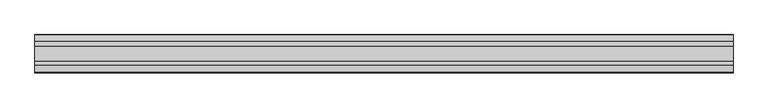
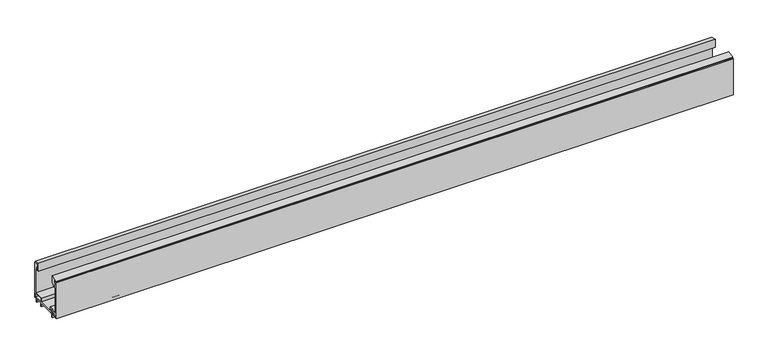
"""IFC4 building model written with IfcOpenShell, lengths in millimetres: proxy geometry, Generic Models 3:Generic Models 2:312240:Generic Models 2:312240 : Generic Models 3:Generic Models 2:312240:21 : Generic Models 3:Generic Models 2:312240:Generic Models 2:312240 : Generic Models 3:Generic Models 2:312240:300533."""

from ifc_helpers import new_model, si_unit, frame, origin, place, context, project, spatial, polyline, outline, extrude, source, transform, mapped, element, save


def generic_models_bb2c0e95(model_context):
    return source(origin(), model_context, "Body", "SweptSolid", [
        extrude(outline(polyline([(-579089.3927119, 38.4543134), (-579089.3434673, 37.5044445), (-579090.0840224, 37.0107412), (-579091.0973491, 37.6694036), (-579092.5052258, 37.6694036), (-579092.5052258, 35.3570787), (-579095.6476161, 35.3570787), (-579095.6476161, 99.8650152), (-579090.1929009, 99.8650152), (-579090.1929009, 96.7226249), (-579091.9716123, 96.426173), (-579090.1929009, 91.5643616), (-579090.1929009, 87.295454), (-579092.5052258, 87.295454), (-579092.5052258, 42.7683765), (-579080.3506973, 42.7683765), (-579080.3506973, 41.3962277), (-579090.2521912, 39.9817285), (-579090.2521912, 38.9309415), (-579089.3927119, 38.4543134)])), frame((591598.4983953, 0.0, 0.0), z_axis=(1.0, 0.0, 0.0), x_axis=(0.0, 1.0, 0.0)), (0.0, 0.0, 1.0), 1150.6736578),
        extrude(outline(polyline([(-579094.0351774, 101.101348), (-579082.6037319, 104.1497335), (-579082.6037319, 92.5441205), (-579088.6970113, 87.295454), (-579089.9023153, 87.295454), (-579089.9023153, 91.8245902), (-579091.4443521, 96.039491), (-579089.9023153, 96.2964971), (-579089.9023153, 100.0627349), (-579094.0351774, 100.0627349), (-579094.0351774, 101.101348)])), frame((591598.4983953, 0.0, 0.0), z_axis=(1.0, 0.0, 0.0), x_axis=(0.0, 1.0, 0.0)), (0.0, 0.0, 1.0), 1150.6736578),
        extrude(outline(polyline([(-579034.6971025, 88.0069386), (-579039.262462, 88.0069386), (-579039.262462, 90.0525332), (-579037.9580736, 91.3568057), (-579037.9580736, 89.5484886), (-579036.475814, 89.5484886), (-579035.4819937, 91.2698359), (-579035.4819937, 93.551255), (-579036.3674154, 95.450048), (-579037.9580736, 95.450048), (-579037.9580736, 93.4168245), (-579039.262462, 93.639525), (-579039.262462, 98.6792075), (-579032.1476161, 98.0807625), (-579032.1476161, 35.6535306), (-579035.7050391, 35.6535306), (-579035.7050391, 29.36875), (-579037.7209121, 29.36875), (-579037.7209121, 35.6535306), (-579048.6303425, 35.6535306), (-579048.6303425, 29.36875), (-579050.6462155, 29.36875), (-579050.6462155, 35.6535306), (-579081.7143761, 35.6535306), (-579081.7143761, 29.36875), (-579083.7302491, 29.36875), (-579083.7302491, 35.6535306), (-579092.3273546, 35.6535306), (-579092.3273546, 37.0172094), (-579091.4972893, 37.5508228), (-579090.5486432, 36.8986286), (-579083.7302491, 36.8986286), (-579082.4258607, 38.203017), (-579078.6905666, 38.203017), (-579078.6905666, 43.5391515), (-579092.1494835, 43.5391515), (-579092.1494835, 45.0807014), (-579076.6746936, 45.0807014), (-579076.6746936, 38.203017), (-579050.7647963, 38.203017), (-579050.7647963, 45.0807014), (-579034.6971025, 45.0807014), (-579034.6971025, 88.0069386)]), holes=[polyline([(-579035.2900064, 37.7879844), (-579035.2900064, 43.5391515), (-579048.6303425, 43.5391515), (-579048.6303425, 37.7879844), (-579035.2900064, 37.7879844)])]), frame((591598.4983953, 0.0, 0.0), z_axis=(1.0, 0.0, 0.0), x_axis=(0.0, 1.0, 0.0)), (0.0, 0.0, 1.0), 1150.6736578),
        extrude(outline(polyline([(-579042.6037319, 102.6595575), (-579032.6450924, 100.4407933), (-579032.6450924, 98.3393783), (-579039.5693075, 98.9217889), (-579039.5693075, 93.4814891), (-579037.6456554, 93.1530607), (-579037.6456554, 95.1913241), (-579036.6213064, 95.1913241), (-579035.7812608, 93.3898405), (-579035.7812608, 91.309542), (-579036.6417092, 89.8192017), (-579037.7308961, 89.8192017), (-579037.7308961, 92.0735899), (-579039.5693075, 90.2351786), (-579039.5693075, 88.0069386), (-579042.6037319, 88.0069386), (-579042.6037319, 102.6595575)])), frame((591598.4983953, 0.0, 0.0), z_axis=(1.0, 0.0, 0.0), x_axis=(0.0, 1.0, 0.0)), (0.0, 0.0, 1.0), 1150.6736578),
    ])


if __name__ == "__main__":
    model = new_model("IFC4")
    model_context = context("Model", 3, world=origin())
    ifc_project = project(units=[si_unit("LENGTHUNIT", "METRE", prefix="MILLI")], contexts=[model_context])
    site = spatial("IfcSite", under=ifc_project)
    building = spatial("IfcBuilding", under=site)
    placement = place(None, origin())
    generic_models_shape = generic_models_bb2c0e95(model_context)
    element("IfcBuildingElementProxy", 1, Name="Generic Models 3:Generic Models 2:312240:Generic Models 2:312240 : Generic Models 3:Generic Models 2:312240:21 : Generic Models 3:Generic Models 2:312240:Generic Models 2:312240 : Generic Models 3:Generic Models 2:312240:300533", ObjectType="Generic Models 3:Generic Models 2:312240:Generic Models 2:312240 : Generic Models 3:Generic Models 2:312240:21 : Generic Models 3:Generic Models 2:312240:Generic Models 2:312240 : Generic Models 3:Generic Models 2:312240:300533", at=placement, inside=building, context=model_context, shape_type="MappedRepresentation", body=[
        mapped(generic_models_shape, transform((0.0, 0.0, 0.0), x_axis=(1.0, 0.0, 0.0), y_axis=(0.0, 1.0, 0.0), z_axis=(0.0, 0.0, 1.0))),
    ])
    save(model, "model.ifc")

# Revit data of these elements
# Type "Generic Models 3:Generic Models 2:312240:Generic Models 2:312240 : Generic Models 3:Generic Models 2:312240:21 : Generic Models 3:Generic Models 2:312240:Generic Models 2:312240 : Generic Models 3:Generic Models 2:312240:300533"
#   NameOverride = "Generic Models 3:Generic Models 2:312240:Generic Models 2:312240 : Generic Models 3:Generic Models 2:312240:300533"
#   ObjectTypeOverride = "Generic Models 2:312240 : Generic Models 3:Generic Models 2:312240"
#   Reference = "Generic Models 2"
#   Tag = "300533"
# Element 1 (IfcBuildingElementProxy, "Generic Models 3:Generic Models 2:312240:Generic Models 2:312240 : Generic Models 3:Generic Models 2:312240:21 : Generic Models 3:Generic Models 2:312240:Generic Models 2:312240 : Generic Models 3:Generic Models 2:312240:300533")
#   Materials on its faces: "THERMAL BROKEN ALUMINUM STOREFRONT FOR POLYCARBONATE"
# Materials
#   "THERMAL BROKEN ALUMINUM STOREFRONT FOR POLYCARBONATE": class "Unassigned", colour RGB 244 244 244, transparency 0, Keynote = "M07611300.01", Cost = 0
